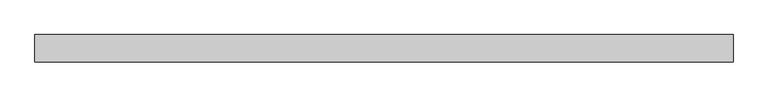
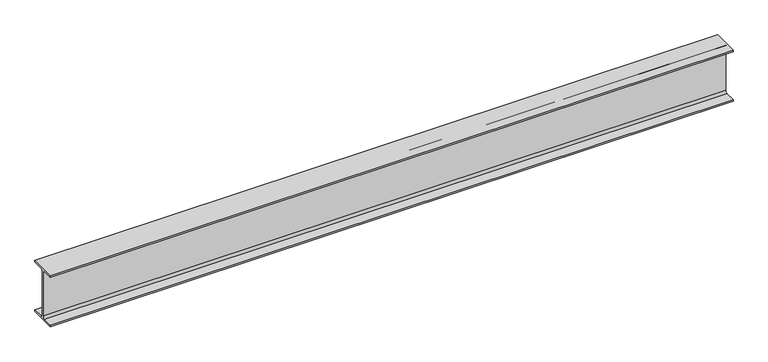
"""IFC4 building model written with IfcOpenShell, lengths in millimetres: beam geometry, 0912_Steel Framing_H-KSD3502 : H_SB_AR_S02_H-300x150x6.5x9_Stair."""

from ifc_helpers import new_model, si_unit, point, frame, frame_2d, origin, place, context, project, spatial, polyline, circle_curve, trimmed, segment, composite_curve, outline, extrude, source, transform, mapped, element, save


def beam_c38fbaf3(model_context):
    return source(origin(), model_context, "Body", "SweptSolid", [
        extrude(outline(composite_curve([segment(polyline([(75.0, -141.0), (75.0, -150.0), (-75.0, -150.0), (-75.0, -141.0), (-16.25, -141.0)]), True, "CONTINUOUS"), segment(trimmed(circle_curve(frame_2d((-16.25, -128.0)), 13.0), [point((-16.25, -141.0))], [point((-3.25, -128.0))], True, "CARTESIAN"), True, "CONTINUOUS"), segment(polyline([(-3.25, -128.0), (-3.25, 128.0)]), True, "CONTINUOUS"), segment(trimmed(circle_curve(frame_2d((-16.25, 128.0)), 13.0), [point((-3.25, 128.0))], [point((-16.25, 141.0))], True, "CARTESIAN"), True, "CONTINUOUS"), segment(polyline([(-16.25, 141.0), (-75.0, 141.0), (-75.0, 150.0), (75.0, 150.0), (75.0, 141.0), (16.25, 141.0)]), True, "CONTINUOUS"), segment(trimmed(circle_curve(frame_2d((16.25, 128.0)), 13.0), [point((16.25, 141.0))], [point((3.25, 128.0))], True, "CARTESIAN"), True, "CONTINUOUS"), segment(polyline([(3.25, 128.0), (3.25, -128.0)]), True, "CONTINUOUS"), segment(trimmed(circle_curve(frame_2d((16.25, -128.0)), 13.0), [point((3.25, -128.0))], [point((16.25, -141.0))], True, "CARTESIAN"), True, "CONTINUOUS"), segment(polyline([(16.25, -141.0), (75.0, -141.0)]), True, "CONTINUOUS")], self_intersect=False)), frame((-1923.1429107, 0.0, 0.0), z_axis=(1.0, 0.0, 0.0), x_axis=(0.0, 1.0, 0.0)), (0.0, 0.0, 1.0), 3799.338853),
    ])


if __name__ == "__main__":
    model = new_model("IFC4")
    model_context = context("Model", 3, world=origin())
    ifc_project = project(units=[si_unit("LENGTHUNIT", "METRE", prefix="MILLI")], contexts=[model_context])
    site = spatial("IfcSite", under=ifc_project)
    building = spatial("IfcBuilding", under=site)
    placement = place(None, origin())
    beam_shape = beam_c38fbaf3(model_context)
    element("IfcBeam", 1, ObjectType="0912_Steel Framing_H-KSD3502 : H_SB_AR_S02_H-300x150x6.5x9_Stair", at=placement, inside=building, context=model_context, shape_type="MappedRepresentation", body=[
        mapped(beam_shape, transform((0.0, 0.0, 0.0), x_axis=(1.0, 0.0, 0.0), y_axis=(0.0, 1.0, 0.0), z_axis=(0.0, 0.0, 1.0))),
    ])
    save(model, "model.ifc")

# Revit data of these elements
# Type "0912_Steel Framing_H-KSD3502 : H_SB_AR_S02_H-300x150x6.5x9_Stair"
#   H_Q'ty Cal Type Tag = "SB-Q2"
#   H_WM Code_1 = "S01AA073-00001 |  | TON | Main Steel Structure Fabrication Work | Shelter/Building | Medium Steel - Standard |  |  |  |  |  |  | Material: (   ) | (90)KG/M>Weight≥(30)KG/M | S01AA073-00001 Main Steel Structure Fabrication Work Shelter/Building Medium Steel - Standard         | - Material: ( ASTM A36 )\n- (90)KG/M>Weight≥(30)KG/M"
#   H_WM Code_2 = "S03AA083-00001 |  | TON | Main Steel Structure Erection Work | Shelter/Building | Medium Steel |  |  |  |  |  |  | Material: (   ) | S03AA083-00001 Main Steel Structure Erection Work Shelter/Building Medium Steel         | - Material: ( ASTM A36 )"
#   H_WM Code_3 = "S01AA009-00001 |  | TON | Main Steel Structure Fabrication Work | Shelter/Building | Plates - Gusset, Stiffener, ETC | Material: (   ) | S01AA009-00001 Main Steel Structure Fabrication Work Shelter/Building Plates - Gusset, Stiffener, ETC         |"
#   H_WM Code_4 = "S41AA051-00001 |  | M2 | Steel Structure Paint Work | Shelter/Building | for Non-Fireproofed Steel Surface |  |  |  |  |  |  | Material: (   ) | S41AA051-00001 Steel Structure Paint Work Shelter/Building for Non-Fireproofed Steel Surface         |"
#   Width = 15.0 cm
#   Web Thickness = 0.65 cm
#   Web Fillet = 1.3 cm
#   Warping Constant = 107000.0 cm⁶
#   W = 0
#   Torsional Moment of Inertia = 9.9539 cm⁴
#   Section Area = 46.78 cm²
#   Plastic Modulus weak axis = 105.0 cm³
#   Plastic Modulus strong axis = 542.0 cm³
#   Perimeter = 1.17 m²/m
#   Nominal Weight = 36.70 kgf/m
#   Moment of Inertia weak axis = 508.00 cm⁴
#   Moment of Inertia strong axis = 7210.00 cm⁴
#   Height = 30.0 cm
#   Flange Thickness = 0.9 cm
#   Elastic Modulus weak axis = 67.7 cm³
#   Elastic Modulus strong axis = 481.0 cm³
#   Centroid Vertical = 15.0 cm
#   Centroid Horizontal = 7.5 cm
#   Ix = 72100000
#   Length [instance default] = 1524 mm
#   Zx = 542000
#   b = 150 mm
#   h = 300 mm
#   r = 13 mm
#   s = 6.5 mm
#   t = 9 mm
#   A = 0.004678 m²
#   Structural Material [instance default] = Steel, 45-345
#   Assembly Code = ""
# Element 1 (IfcBeam, "0912_Steel Framing_H-KSD3502 : H_SB_AR_S02_H-300x150x6.5x9_Stair")
#   Materials on its faces: "Steel, 45-345"
# Materials
#   "Steel, 45-345": class "Metal", colour RGB 189 187 185, transparency 0, Description = "Steel 345 MPa", Cost = 0
